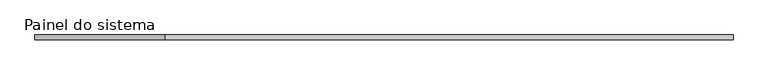
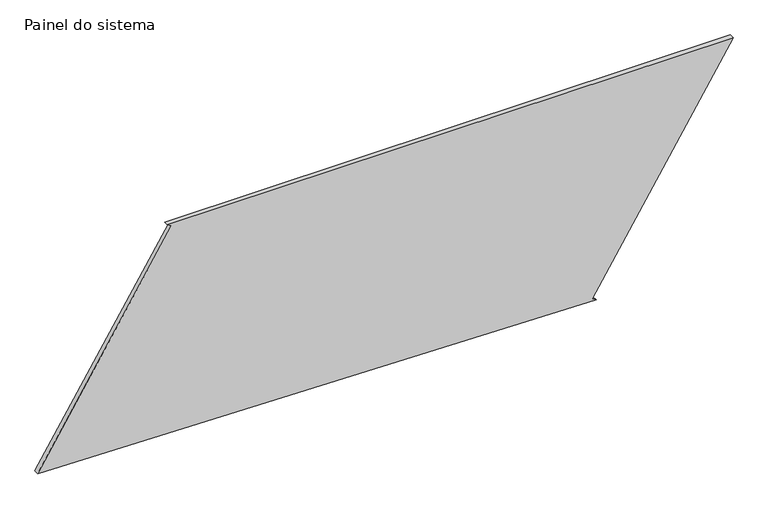
"""IFC4 building model written with IfcOpenShell, lengths in millimetres: plate geometry, Painel do sistema : Envidraçado."""

from ifc_helpers import new_model, si_unit, frame, origin, place, context, project, spatial, polyline, outline, extrude, source, transform, mapped, element, save


def painel_do_sistema_a5ca431a(model_context):
    return source(origin(), model_context, "Body", "SweptSolid", [
        extrude(outline(polyline([(0.0, 1117.2094057), (13.2016257, 1095.9793073), (1216.0258348, 1843.9379218), (1216.0258348, -1156.0822479), (1202.8242091, -1134.8521495), (62.5130787, -1843.9379218), (0.0, 1117.2094057)])), frame((0.0, 24.5, 0.0), z_axis=(0.0, 1.0, 0.0), x_axis=(0.0, 0.0, 1.0)), (0.0, 0.0, 1.0), 25.0),
    ])


if __name__ == "__main__":
    model = new_model("IFC4")
    model_context = context("Model", 3, world=origin())
    ifc_project = project(units=[si_unit("LENGTHUNIT", "METRE", prefix="MILLI")], contexts=[model_context])
    site = spatial("IfcSite", under=ifc_project)
    building = spatial("IfcBuilding", under=site)
    placement = place(None, origin())
    painel_do_sistema_shape = painel_do_sistema_a5ca431a(model_context)
    element("IfcPlate", 1, ObjectType="Painel do sistema : Envidraçado", at=placement, inside=building, context=model_context, shape_type="MappedRepresentation", body=[
        mapped(painel_do_sistema_shape, transform((0.0, 0.0, 0.0), x_axis=(1.0, 0.0, 0.0), y_axis=(0.0, 1.0, 0.0), z_axis=(0.0, 0.0, 1.0))),
    ])
    save(model, "model.ifc")

# Revit data of these elements
# Type "Painel do sistema : Envidraçado"
#   Construction Type Id = "GSP4R"
#   Analytic Construction = "Vidraça única Pilkington 1/8 pol"
#   Visual Light Transmittance = 0.9
#   Solar Heat Gain Coefficient = 0.86
#   Heat Transfer Coefficient (U) = 6.7069 W/(m²·K)
# Element 1 (IfcPlate, "Painel do sistema : Envidraçado")
#   Materials on its faces: "Vidro"
# Materials
#   "Vidro": class "Vidro", colour RGB 0 128 192, transparency 0.9, Description = "Vidro de sílica", Cost = 0
